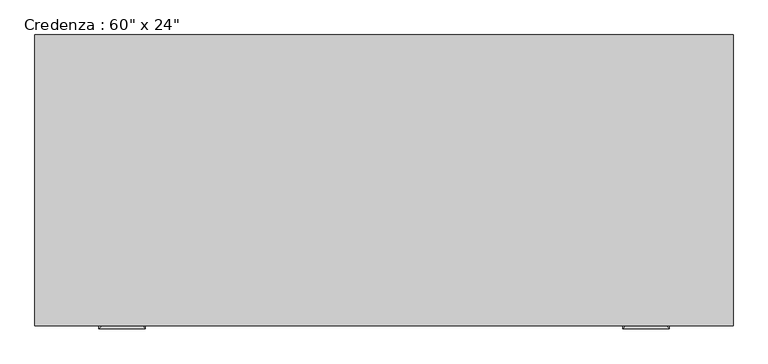
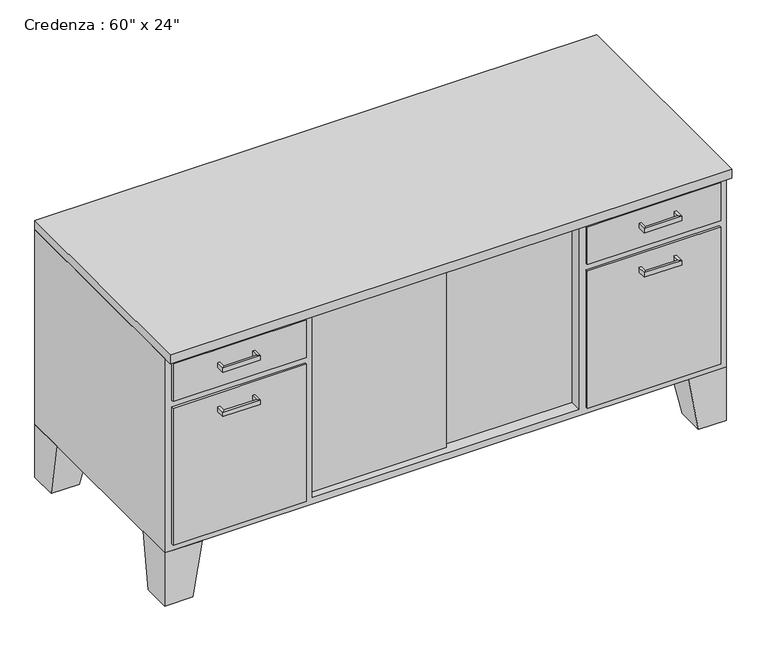
"""IFC4 building model written with IfcOpenShell, lengths in millimetres: furniture geometry."""

from ifc_helpers import new_model, si_unit, frame, origin, place, context, project, spatial, polyline, outline, extrude, faceted_brep, source, transform, mapped, element, save


def furniture_0f0bb7e9(model_context):
    return source(origin(), model_context, "Body", "SolidModel", [
        extrude(outline(polyline([(455.5023176, -267.2714583), (46.8442623, -267.2714583), (46.8442623, -254.5714583), (455.5023176, -254.5714583), (455.5023176, -267.2714583)])), frame((0.0, 0.0, 171.45), z_axis=(0.0, 0.0, 1.0), x_axis=(1.0, 0.0, 0.0)), (0.0, 0.0, 1.0), 520.7),
        extrude(outline(polyline([(73.6254475, -279.9714583), (-302.4057377, -279.9714583), (-302.4057377, -267.2714583), (73.6254475, -267.2714583), (73.6254475, -279.9714583)])), frame((0.0, 0.0, 171.45), z_axis=(0.0, 0.0, 1.0), x_axis=(1.0, 0.0, 0.0)), (0.0, 0.0, 1.0), 520.7),
        faceted_brep([(719.9442623, 309.3803279, 152.4), (719.9442623, 207.7803279, 152.4), (821.5442623, 207.7803279, 152.4), (821.5442623, 309.3803279, 152.4), (745.3442623, 309.3803279, 0.0), (821.5442623, 309.3803279, 0.0), (821.5442623, 233.1803279, 0.0), (745.3442623, 233.1803279, 0.0)], [[[0, 1, 2, 3]], [[4, 5, 6, 7]], [[4, 7, 1, 0]], [[7, 6, 2, 1]], [[6, 5, 3, 2]], [[5, 4, 0, 3]]]),
        extrude(outline(polyline([(802.4942623, -306.5696721), (440.5442623, -306.5696721), (440.5442623, -300.2196721), (802.4942623, -300.2196721), (802.4942623, -306.5696721)])), frame((0.0, 0.0, 584.2), z_axis=(0.0, 0.0, 1.0), x_axis=(1.0, 0.0, 0.0)), (0.0, 0.0, 1.0), 107.95),
        extrude(outline(polyline([(802.4942623, -306.5696721), (440.5442623, -306.5696721), (440.5442623, -300.2196721), (802.4942623, -300.2196721), (802.4942623, -306.5696721)])), frame((0.0, 0.0, 171.45), z_axis=(0.0, 0.0, 1.0), x_axis=(1.0, 0.0, 0.0)), (0.0, 0.0, 1.0), 393.7),
        extrude(outline(polyline([(-321.4557377, -306.5696721), (-683.4057377, -306.5696721), (-683.4057377, -300.2196721), (-321.4557377, -300.2196721), (-321.4557377, -306.5696721)])), frame((0.0, 0.0, 584.2), z_axis=(0.0, 0.0, 1.0), x_axis=(1.0, 0.0, 0.0)), (0.0, 0.0, 1.0), 107.95),
        extrude(outline(polyline([(-321.4557377, -306.5696721), (-683.4057377, -306.5696721), (-683.4057377, -300.2196721), (-321.4557377, -300.2196721), (-321.4557377, -306.5696721)])), frame((0.0, 0.0, 171.45), z_axis=(0.0, 0.0, 1.0), x_axis=(1.0, 0.0, 0.0)), (0.0, 0.0, 1.0), 393.7),
        faceted_brep([(-600.8557377, -300.2196721, 152.4), (-600.8557377, -198.6196721, 152.4), (-702.4557377, -198.6196721, 152.4), (-702.4557377, -300.2196721, 152.4), (-626.2557377, -300.2196721, 0.0), (-702.4557377, -300.2196721, 0.0), (-702.4557377, -224.0196721, 0.0), (-626.2557377, -224.0196721, 0.0)], [[[0, 1, 2, 3]], [[4, 5, 6, 7]], [[4, 7, 1, 0]], [[7, 6, 2, 1]], [[6, 5, 3, 2]], [[5, 4, 0, 3]]]),
        faceted_brep([(-600.8557377, 309.3803279, 152.4), (-702.4557377, 309.3803279, 152.4), (-702.4557377, 207.7803279, 152.4), (-600.8557377, 207.7803279, 152.4), (-626.2557377, 309.3803279, 0.0), (-626.2557377, 233.1803279, 0.0), (-702.4557377, 233.1803279, 0.0), (-702.4557377, 309.3803279, 0.0)], [[[0, 1, 2, 3]], [[4, 5, 6, 7]], [[4, 7, 1, 0]], [[7, 6, 2, 1]], [[6, 5, 3, 2]], [[5, 4, 0, 3]]]),
        faceted_brep([(719.9442623, -300.2196721, 152.4), (821.5442623, -300.2196721, 152.4), (821.5442623, -198.6196721, 152.4), (719.9442623, -198.6196721, 152.4), (745.3442623, -300.2196721, 0.0), (745.3442623, -224.0196721, 0.0), (821.5442623, -224.0196721, 0.0), (821.5442623, -300.2196721, 0.0)], [[[0, 1, 2, 3]], [[4, 5, 6, 7]], [[4, 7, 1, 0]], [[7, 6, 2, 1]], [[6, 5, 3, 2]], [[5, 4, 0, 3]]]),
        faceted_brep([(821.5442623, 309.3803279, 711.2), (-702.4557377, 309.3803279, 711.2), (-702.4557377, -300.2196721, 711.2), (821.5442623, -300.2196721, 711.2), (821.5442623, 309.3803279, 152.4), (821.5442623, -300.2196721, 152.4), (-702.4557377, -300.2196721, 152.4), (-702.4557377, 309.3803279, 152.4), (-302.4057377, -300.2196721, 692.15), (421.4942623, -300.2196721, 692.15), (421.4942623, -300.2196721, 171.45), (-302.4057377, -300.2196721, 171.45), (421.4942623, 290.3303279, 692.15), (-302.4057377, 290.3303279, 692.15), (-302.4057377, 290.3303279, 171.45), (421.4942623, 290.3303279, 171.45)], [[[0, 1, 2, 3]], [[4, 5, 6, 7]], [[1, 0, 4, 7]], [[2, 1, 7, 6]], [[3, 2, 6, 5], [8, 9, 10, 11]], [[0, 3, 5, 4]], [[12, 13, 14, 15]], [[13, 12, 9, 8]], [[14, 13, 8, 11]], [[15, 14, 11, 10]], [[12, 15, 10, 9]]]),
        extrude(outline(polyline([(821.5442623, 309.3803279), (821.5442623, -325.6196721), (-702.4557377, -325.6196721), (-702.4557377, 309.3803279), (821.5442623, 309.3803279)])), frame((0.0, 0.0, 711.2), z_axis=(0.0, 0.0, 1.0), x_axis=(1.0, 0.0, 0.0)), (0.0, 0.0, 1.0), 25.4),
        faceted_brep([(-556.4057377, -306.5696721, 527.05), (-556.4057377, -306.5696721, 514.35), (-562.7557377, -306.5696721, 514.35), (-562.7557377, -306.5696721, 527.05), (-556.4057377, -325.6196721, 527.05), (-556.4057377, -325.6196721, 514.35), (-562.7557377, -331.9696721, 514.35), (-562.7557377, -331.9696721, 527.05), (-467.5057377, -325.6196721, 527.05), (-467.5057377, -325.6196721, 514.35), (-461.1557377, -331.9696721, 514.35), (-461.1557377, -331.9696721, 527.05), (-467.5057377, -306.5696721, 527.05), (-461.1557377, -306.5696721, 527.05), (-461.1557377, -306.5696721, 514.35), (-467.5057377, -306.5696721, 514.35)], [[[0, 1, 2, 3]], [[1, 0, 4, 5]], [[2, 1, 5, 6]], [[3, 2, 6, 7]], [[0, 3, 7, 4]], [[5, 4, 8, 9]], [[6, 5, 9, 10]], [[7, 6, 10, 11]], [[4, 7, 11, 8]], [[12, 13, 14, 15]], [[9, 8, 12, 15]], [[10, 9, 15, 14]], [[11, 10, 14, 13]], [[8, 11, 13, 12]]]),
        faceted_brep([(-556.4057377, -306.5696721, 654.05), (-556.4057377, -306.5696721, 641.35), (-562.7557377, -306.5696721, 641.35), (-562.7557377, -306.5696721, 654.05), (-556.4057377, -325.6196721, 654.05), (-556.4057377, -325.6196721, 641.35), (-562.7557377, -331.9696721, 641.35), (-562.7557377, -331.9696721, 654.05), (-467.5057377, -325.6196721, 654.05), (-467.5057377, -325.6196721, 641.35), (-461.1557377, -331.9696721, 641.35), (-461.1557377, -331.9696721, 654.05), (-467.5057377, -306.5696721, 654.05), (-461.1557377, -306.5696721, 654.05), (-461.1557377, -306.5696721, 641.35), (-467.5057377, -306.5696721, 641.35)], [[[0, 1, 2, 3]], [[1, 0, 4, 5]], [[2, 1, 5, 6]], [[3, 2, 6, 7]], [[0, 3, 7, 4]], [[5, 4, 8, 9]], [[6, 5, 9, 10]], [[7, 6, 10, 11]], [[4, 7, 11, 8]], [[12, 13, 14, 15]], [[9, 8, 12, 15]], [[10, 9, 15, 14]], [[11, 10, 14, 13]], [[8, 11, 13, 12]]]),
        faceted_brep([(586.5942623, -306.5696721, 654.1373112), (586.5942623, -306.5696721, 641.4373112), (580.2442623, -306.5696721, 641.4373112), (580.2442623, -306.5696721, 654.1373112), (586.5942623, -325.6196721, 654.1373112), (586.5942623, -325.6196721, 641.4373112), (580.2442623, -331.9696721, 641.4373112), (580.2442623, -331.9696721, 654.1373112), (675.4942623, -325.6196721, 654.1373112), (675.4942623, -325.6196721, 641.4373112), (681.8442623, -331.9696721, 641.4373112), (681.8442623, -331.9696721, 654.1373112), (675.4942623, -306.5696721, 654.1373112), (681.8442623, -306.5696721, 654.1373112), (681.8442623, -306.5696721, 641.4373112), (675.4942623, -306.5696721, 641.4373112)], [[[0, 1, 2, 3]], [[1, 0, 4, 5]], [[2, 1, 5, 6]], [[3, 2, 6, 7]], [[0, 3, 7, 4]], [[5, 4, 8, 9]], [[6, 5, 9, 10]], [[7, 6, 10, 11]], [[4, 7, 11, 8]], [[12, 13, 14, 15]], [[9, 8, 12, 15]], [[10, 9, 15, 14]], [[11, 10, 14, 13]], [[8, 11, 13, 12]]]),
        faceted_brep([(586.5942623, -306.5696721, 527.05), (586.5942623, -306.5696721, 514.35), (580.2442623, -306.5696721, 514.35), (580.2442623, -306.5696721, 527.05), (586.5942623, -325.6196721, 527.05), (586.5942623, -325.6196721, 514.35), (580.2442623, -331.9696721, 514.35), (580.2442623, -331.9696721, 527.05), (675.4942623, -325.6196721, 527.05), (675.4942623, -325.6196721, 514.35), (681.8442623, -331.9696721, 514.35), (681.8442623, -331.9696721, 527.05), (675.4942623, -306.5696721, 527.05), (681.8442623, -306.5696721, 527.05), (681.8442623, -306.5696721, 514.35), (675.4942623, -306.5696721, 514.35)], [[[0, 1, 2, 3]], [[1, 0, 4, 5]], [[2, 1, 5, 6]], [[3, 2, 6, 7]], [[0, 3, 7, 4]], [[5, 4, 8, 9]], [[6, 5, 9, 10]], [[7, 6, 10, 11]], [[4, 7, 11, 8]], [[12, 13, 14, 15]], [[9, 8, 12, 15]], [[10, 9, 15, 14]], [[11, 10, 14, 13]], [[8, 11, 13, 12]]]),
    ])


if __name__ == "__main__":
    model = new_model("IFC4")
    model_context = context("Model", 3, world=origin())
    ifc_project = project(units=[si_unit("LENGTHUNIT", "METRE", prefix="MILLI")], contexts=[model_context])
    site = spatial("IfcSite", under=ifc_project)
    building = spatial("IfcBuilding", under=site)
    placement = place(None, origin())
    furniture_shape = furniture_0f0bb7e9(model_context)
    element("IfcFurniture", 1, ObjectType="Credenza : 60\" x 24\"", at=placement, inside=building, context=model_context, shape_type="MappedRepresentation", body=[
        mapped(furniture_shape, transform((0.0, 0.0, 0.0), x_axis=(1.0, 0.0, 0.0), y_axis=(0.0, 1.0, 0.0), z_axis=(0.0, 0.0, 1.0))),
    ])
    save(model, "model.ifc")

# Revit data of these elements
# Type "Credenza : 60\" x 24\""
#   Assembly Code = "E2020200"
#   Depth = 2' - 0"
#   Height = 2' - 5"
#   Width = 5' - 0"
#   Body Material = Laminate, Ivory, Matte
#   Handles/Legs Material = Steel, Chrome Plated
#   Top Material = Cherry
#   Default Elevation = 0
# Element 1 (IfcFurniture, "Credenza : 60\" x 24\"")
#   Materials on its faces: "Steel, Chrome Plated", "Laminate, Ivory, Matte", "Cherry"
# Materials
#   "Laminate, Ivory, Matte": class "Plastic", colour RGB 247 247 239, transparency 0, Description = "Plastic Laminate - Ivory, Matte", Cost = 0
#   "Steel, Chrome Plated": class "Metal", colour RGB 17 17 17, transparency 0, Description = "Chromiuim plated steel", Cost = 0
#   "Cherry": class "Wood", colour RGB 226 177 128, transparency 0, Description = "Prunus Serotina", Cost = 0
